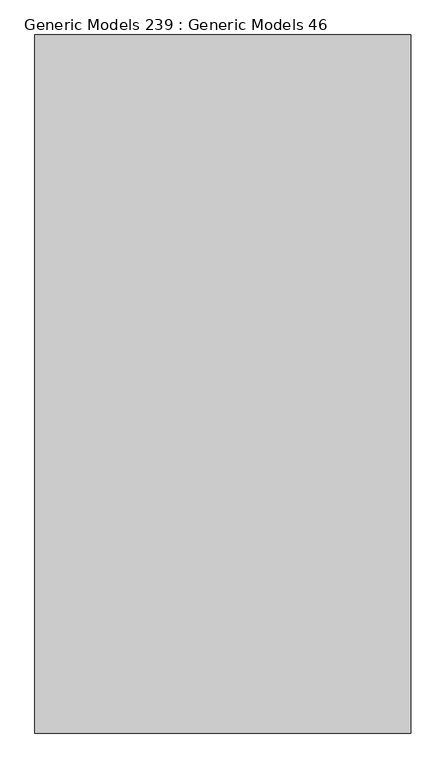
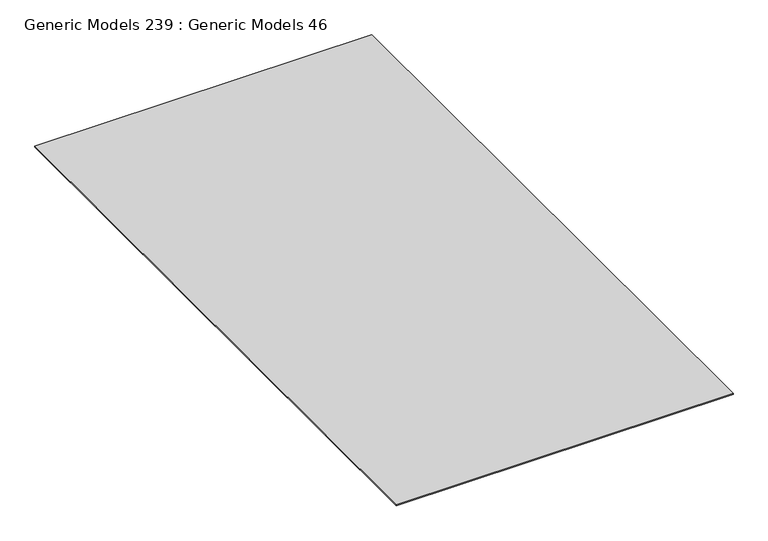
"""IFC4 building model written with IfcOpenShell, lengths in millimetres: proxy geometry, Generic Models 239 : Generic Models 46."""

import ifcopenshell
import ifcopenshell.guid

model = None  # the IFC model being written
_history = None  # IfcOwnerHistory: only IFC2X3 demands one
_inside = {}  # id of a spatial element -> (the spatial element, [elements in it])
_under = {}  # id of a project, library or spatial element -> (it, [spatial elements below it])
_declared = {}  # id of a project -> (the project, [libraries it declares])
_typed = {}  # id of a type object -> (the type object, [elements of that type])
_made_of = {}  # id of a material, layer set ... -> (it, [elements and type objects made of it])


def new_model(schema):
    """Start an empty IFC model of exactly this schema.

    Asked for "IFC4X3", IfcOpenShell would pick the latest addendum, in which some entities
    have other attributes; the version numbers below select the first issue.
    IFC2X3 requires an IfcOwnerHistory on every rooted entity: one is made here for all.
    """
    global model, _history
    if schema == "IFC4X3":
        model = ifcopenshell.file(schema_version=(4, 3, 0, 0))
    else:
        model = ifcopenshell.file(schema=schema)
    _inside.clear()
    _under.clear()
    _declared.clear()
    _typed.clear()
    _made_of.clear()
    _history = None
    if model.schema == "IFC2X3":
        org = make("IfcOrganization", Name="unknown")
        user = make(
            "IfcPersonAndOrganization",
            ThePerson=make("IfcPerson", FamilyName="unknown"),
            TheOrganization=org,
        )
        app = make(
            "IfcApplication",
            ApplicationDeveloper=org,
            Version="unknown",
            ApplicationFullName="unknown",
            ApplicationIdentifier="unknown",
        )
        _history = make(
            "IfcOwnerHistory",
            OwningUser=user,
            OwningApplication=app,
            ChangeAction="ADDED",
            CreationDate=0,
        )
    return model


def make(cls, **values):
    """One entity of the class cls with the attributes given. An attribute that is None is left unset."""
    return model.create_entity(
        cls, **{name: value for name, value in values.items() if value is not None}
    )


def rooted(cls, **values):
    """An entity with a GlobalId (a new one), such as an element, a storey or a relation."""
    return make(cls, GlobalId=ifcopenshell.guid.new(), OwnerHistory=_history, **values)


def si_unit(unit_type, name, prefix=None):
    """IfcSIUnit, for example si_unit("LENGTHUNIT", "METRE", prefix="MILLI")."""
    return make("IfcSIUnit", UnitType=unit_type, Prefix=prefix, Name=name)


def assignment(units):
    """IfcUnitAssignment: the units of a project."""
    return None if units is None else make("IfcUnitAssignment", Units=units)


def point(xyz):
    """IfcCartesianPoint."""
    return None if xyz is None else make("IfcCartesianPoint", Coordinates=xyz)


def direction(xyz):
    """IfcDirection."""
    return None if xyz is None else make("IfcDirection", DirectionRatios=xyz)


def frame(location, z_axis=None, x_axis=None):
    """IfcAxis2Placement3D, a coordinate frame: its origin and axes. An axis left out is left unset."""
    return make(
        "IfcAxis2Placement3D",
        Location=point(location),
        Axis=direction(z_axis),
        RefDirection=direction(x_axis),
    )


def origin():
    """The frame at (0, 0, 0) with its axes left unset."""
    return frame((0.0, 0.0, 0.0))


def place(relative_to, where):
    """IfcLocalPlacement: puts the frame where relative to a parent placement (None: the world)."""
    return make(
        "IfcLocalPlacement", PlacementRelTo=relative_to, RelativePlacement=where
    )


def context(
    kind, dimensions, precision=None, world=None, true_north=None, identifier=None
):
    """IfcGeometricRepresentationContext, for example the 3D "Model" context."""
    return make(
        "IfcGeometricRepresentationContext",
        ContextIdentifier=identifier,
        ContextType=kind,
        CoordinateSpaceDimension=dimensions,
        Precision=precision,
        WorldCoordinateSystem=world,
        TrueNorth=true_north,
    )


def project(units=None, contexts=None):
    """IfcProject with its units and contexts."""
    return rooted(
        "IfcProject",
        Name="project",
        RepresentationContexts=contexts,
        UnitsInContext=assignment(units),
    )


def spatial(cls, under=None, at=None, **own):
    """A site, building, storey or space (cls), placed at a placement, below another one or the project."""
    s = rooted(cls, ObjectPlacement=at, **own)
    if under is not None:
        _under.setdefault(under.id(), (under, []))[1].append(s)
    return s


def polyline(points):
    """IfcPolyline through the points."""
    return make("IfcPolyline", Points=[point(p) for p in points])


def outline(outer, holes=None, kind="AREA"):
    """IfcArbitraryClosedProfileDef: a profile drawn as a closed curve; with holes, ...WithVoids."""
    if holes is None:
        return make("IfcArbitraryClosedProfileDef", ProfileType=kind, OuterCurve=outer)
    return make(
        "IfcArbitraryProfileDefWithVoids",
        ProfileType=kind,
        OuterCurve=outer,
        InnerCurves=holes,
    )


def extrude(swept, where, along, depth):
    """IfcExtrudedAreaSolid: the profile swept, set in the frame where, extruded along a direction by depth."""
    return make(
        "IfcExtrudedAreaSolid",
        SweptArea=swept,
        Position=where,
        ExtrudedDirection=direction(along),
        Depth=depth,
    )


def shape(context_of_items, identifier, shape_type, items):
    """IfcShapeRepresentation: the items that make up one representation, for example the "Body"."""
    return make(
        "IfcShapeRepresentation",
        ContextOfItems=context_of_items,
        RepresentationIdentifier=identifier,
        RepresentationType=shape_type,
        Items=items,
    )


def source(mapping_origin, context_of_items, identifier, shape_type, items):
    """IfcRepresentationMap: a shape defined once, which mapped items show again and again."""
    return make(
        "IfcRepresentationMap",
        MappingOrigin=mapping_origin,
        MappedRepresentation=shape(context_of_items, identifier, shape_type, items),
    )


def transform(
    local_origin,
    x_axis=None,
    y_axis=None,
    z_axis=None,
    scale=None,
    scale2=None,
    scale3=None,
    uniform=True,
):
    """IfcCartesianTransformationOperator3D, or its non-uniform kind. x_axis, y_axis, z_axis: its Axis1, 2, 3."""
    if uniform:
        return make(
            "IfcCartesianTransformationOperator3D",
            Axis1=direction(x_axis),
            Axis2=direction(y_axis),
            LocalOrigin=point(local_origin),
            Scale=scale,
            Axis3=direction(z_axis),
        )
    return make(
        "IfcCartesianTransformationOperator3DnonUniform",
        Axis1=direction(x_axis),
        Axis2=direction(y_axis),
        LocalOrigin=point(local_origin),
        Scale=scale,
        Axis3=direction(z_axis),
        Scale2=scale2,
        Scale3=scale3,
    )


def mapped(mapping_source, mapping_target):
    """IfcMappedItem: shows the shape of a source again, moved by a transform."""
    return make(
        "IfcMappedItem", MappingSource=mapping_source, MappingTarget=mapping_target
    )


def made_of(thing, what):
    """Note that an element or type object is made of a material, layer set ...; save() writes the relation."""
    if what is not None:
        _made_of.setdefault(what.id(), (what, []))[1].append(thing)
    return thing


def element(
    cls,
    number,
    at=None,
    inside=None,
    cuts=None,
    type_object=None,
    material=None,
    context=None,
    identifier="Body",
    shape_type=None,
    held_by="IfcProductDefinitionShape",
    body=None,
    shapes=None,
    **own,
):
    """One element of the class cls, such as IfcWall. Its Tag is "e" and its number.

    at: its placement. inside: the storey or other place that contains it. cuts: it is an
    opening in that element (IfcRelVoidsElement). A single representation is given by context,
    identifier, shape_type and body (its items); several are given by shapes. held_by: the class
    of the entity that holds the representations. save() writes the other relations.
    """
    e = rooted(cls, Tag="e%d" % number, ObjectPlacement=at, **own)
    if body is not None:
        shapes = [shape(context, identifier, shape_type, body)]
    if shapes is not None:
        e.Representation = make(held_by, Representations=shapes)
    if inside is not None:
        _inside.setdefault(inside.id(), (inside, []))[1].append(e)
    if cuts is not None:
        rooted(
            "IfcRelVoidsElement", RelatingBuildingElement=cuts, RelatedOpeningElement=e
        )
    if type_object is not None:
        _typed.setdefault(type_object.id(), (type_object, []))[1].append(e)
    return made_of(e, material)


def aggregate(whole, parts):
    """IfcRelAggregates: a whole, such as a stair, and the parts it consists of."""
    return rooted("IfcRelAggregates", RelatingObject=whole, RelatedObjects=parts)


def save(model, path):
    """Write the relations noted so far, then the file.

    IfcRelAggregates (storeys below a building ...), IfcRelContainedInSpatialStructure (elements
    in a storey), IfcRelDefinesByType, IfcRelAssociatesMaterial and IfcRelDeclares: one each for
    every whole, place, type object, material and project.
    """
    for whole, parts in _under.values():
        aggregate(whole, parts)
    for where, things in _inside.values():
        rooted(
            "IfcRelContainedInSpatialStructure",
            RelatedElements=things,
            RelatingStructure=where,
        )
    for kind, things in _typed.values():
        rooted("IfcRelDefinesByType", RelatedObjects=things, RelatingType=kind)
    for what, things in _made_of.values():
        rooted("IfcRelAssociatesMaterial", RelatedObjects=things, RelatingMaterial=what)
    for by, libraries in _declared.values():
        rooted("IfcRelDeclares", RelatingContext=by, RelatedDefinitions=libraries)
    model.write(path)


def generic_models_239_generic_models_46_95e6735a(model_context):
    return source(origin(), model_context, "Body", "SweptSolid", [
        extrude(outline(polyline([(50347.5625, 0.0), (49691.4320511, 0.0), (49691.4320511, 1219.2), (50347.5625, 1219.2), (50347.5625, 0.0)])), frame((0.0, 0.0, 5505.7509163), z_axis=(0.0, 0.0, 1.0), x_axis=(1.0, 0.0, 0.0)), (0.0, 0.0, 1.0), 1.5875),
    ])


if __name__ == "__main__":
    model = new_model("IFC4")
    model_context = context("Model", 3, world=origin())
    ifc_project = project(units=[si_unit("LENGTHUNIT", "METRE", prefix="MILLI")], contexts=[model_context])
    site = spatial("IfcSite", under=ifc_project)
    building = spatial("IfcBuilding", under=site)
    placement = place(None, origin())
    generic_models_239_generic_models_46_shape = generic_models_239_generic_models_46_95e6735a(model_context)
    element("IfcBuildingElementProxy", 1, Name="Generic Models 239 : Generic Models 46", ObjectType="Generic Models 239 : Generic Models 46", at=placement, inside=building, context=model_context, shape_type="MappedRepresentation", body=[
        mapped(generic_models_239_generic_models_46_shape, transform((0.0, 0.0, 0.0), x_axis=(1.0, 0.0, 0.0), y_axis=(0.0, 1.0, 0.0), z_axis=(0.0, 0.0, 1.0))),
    ])
    save(model, "model.ifc")

# Revit data of these elements
# Element 1 (IfcBuildingElementProxy, "Generic Models 239 : Generic Models 46")
#   Materials on its faces: "SET IN BED OF SEALANT"
# Materials
#   "SET IN BED OF SEALANT": class "Unassigned", colour RGB 58 208 21, transparency 0, Cost = 0
